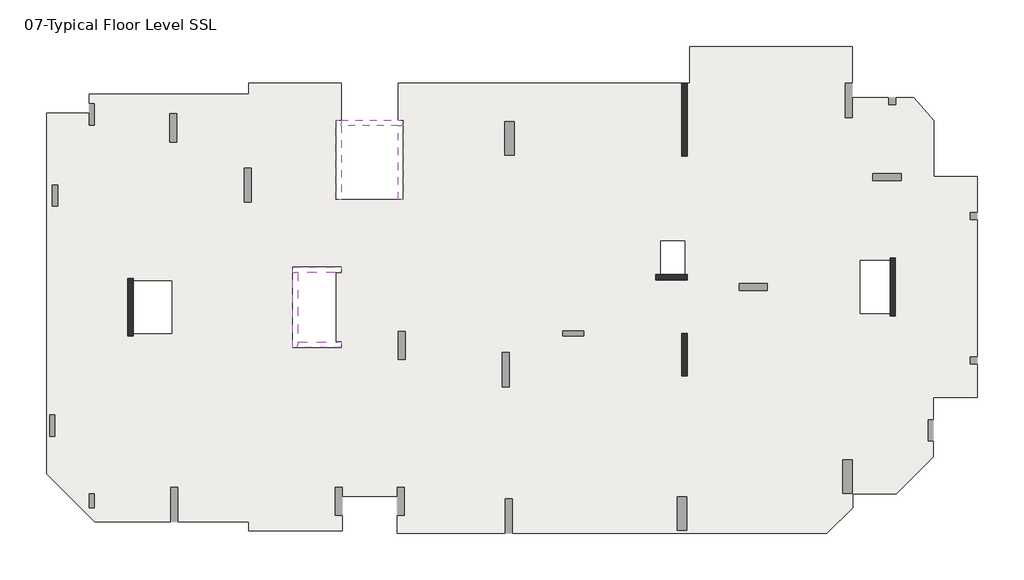
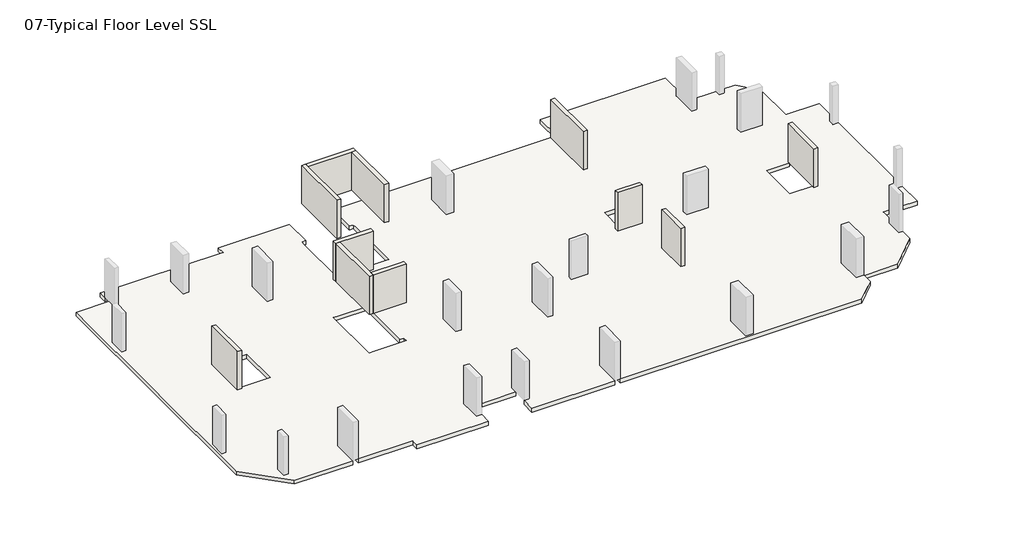
# One storey, part 1 of 2: 11 walls, 1 slab.
"""IFC4 building model written with IfcOpenShell, lengths in millimetres."""

from ifc_helpers import new_model, si_unit, origin, place, context, project, spatial, faceted_brep, element, save

model = new_model("IFC4")

# Units and contexts
model_context = context("Model", 3, world=origin())
ifc_project = project(units=[si_unit("LENGTHUNIT", "METRE", prefix="MILLI")], contexts=[model_context])

# Site, building, storey
site = spatial("IfcSite", under=ifc_project)
building = spatial("IfcBuilding", under=site)
storey = spatial("IfcBuildingStorey", under=building, Name="07-Typical Floor Level SSL", Elevation=15000.0)

# Slab
placement = place(None, origin())
element("IfcSlab", 1, ObjectType="Generic 300mm", at=placement, inside=storey, context=model_context, shape_type="Brep", body=[
    faceted_brep([(36192.0021644, 24072.000519, 14700.0), (36192.0021644, 26172.000519, 14700.0), (45446.0007483, 26172.000519, 14700.0), (45446.0007483, 24087.0, 14700.0), (45046.0007483, 24087.0, 14700.0), (45046.0007483, 22137.0, 14700.0), (45446.0007483, 22137.0, 14700.0), (45446.0007483, 23252.0000315, 14700.0), (47498.6337868, 23252.0000315, 14700.0), (47498.6337868, 22852.0, 14700.0), (47898.6337868, 22852.0, 14700.0), (47898.6337868, 23252.0000315, 14700.0), (48936.764334, 23252.0000315, 14700.0), (50076.0016214, 21956.8283806, 14700.0), (50076.0016214, 18780.0084406, 14700.0), (52549.9999998, 18780.0084406, 14700.0), (52549.9999998, 16712.0, 14700.0), (52149.9999998, 16712.0, 14700.0), (52149.9999998, 16312.0, 14700.0), (52549.9999998, 16312.0, 14700.0), (52549.9999998, 8504.0039609, 14700.0), (52149.9999998, 8504.0039609, 14700.0), (52149.9999998, 8104.0039609, 14700.0), (52549.9999998, 8104.0039609, 14700.0), (52549.9999998, 6204.0084406, 14700.0), (50046.0009271, 6204.0084406, 14700.0), (50046.0009271, 4931.9999929, 14700.0), (49746.0009271, 4931.9999929, 14700.0), (49746.0009271, 3731.9999929, 14700.0), (50046.0009271, 3731.9999929, 14700.0), (50046.0009271, 2810.5958657, 14700.0), (47943.4055804, 708.000519, 14700.0), (45456.0017287, 708.000519, 14700.0), (45456.0017287, -61.7051085, 14700.0), (43990.7023722, -1527.004465, 14700.0), (26113.9999998, -1527.004465, 14700.0), (26113.9999998, 422.995535, 14700.0), (25713.9999998, 422.995535, 14700.0), (25713.9999998, -1527.004465, 14700.0), (19569.9997488, -1527.004465, 14700.0), (19569.9997488, -512.0044652, 14700.0), (19969.9997488, -512.0044652, 14700.0), (19969.9997488, 1087.9955348, 14700.0), (19569.9997488, 1087.9955348, 14700.0), (19569.9997488, 564.000519, 14700.0), (16429.9999981, 564.000519, 14700.0), (16429.9999981, 1088.0, 14700.0), (16029.9999981, 1088.0, 14700.0), (16029.9999981, -512.0, 14700.0), (16429.9999981, -512.0, 14700.0), (16429.9999981, -1391.999481, 14700.0), (11136.0000923, -1391.999481, 14700.0), (11136.0000923, -866.9999847, 14700.0), (7082.0000416, -866.9999847, 14700.0), (7082.0000416, 1083.0000153, 14700.0), (6682.0000416, 1083.0000153, 14700.0), (6682.0000416, -866.9999847, 14700.0), (2364.4419097, -866.9999847, 14700.0), (-372.0, 1869.441925, 14700.0), (-372.0, 22380.0004589, 14700.0), (2052.0, 22380.0004589, 14700.0), (2052.0, 21708.0000656, 14700.0), (2352.0, 21708.0000656, 14700.0), (2352.0, 22908.0000656, 14700.0), (2052.0, 22908.0000656, 14700.0), (2052.0, 23472.000519, 14700.0), (11136.0000923, 23472.000519, 14700.0), (11136.0000923, 24072.000519, 14700.0), (16380.0000168, 24072.000519, 14700.0), (16380.0000168, 21972.0, 14700.0), (16079.9999997, 21972.0, 14700.0), (16079.9999997, 21672.0, 14700.0), (16079.9999997, 17468.0, 14700.0), (16379.9999997, 17468.0, 14700.0), (19619.9999997, 17468.0, 14700.0), (19919.9999997, 17468.0, 14700.0), (19919.9999997, 21672.0, 14700.0), (19919.9999997, 21972.0, 14700.0), (19619.9997365, 21972.0, 14700.0), (19619.9997365, 24072.000519, 14700.0), (35747.9999998, 24072.000519, 14700.0), (35747.9999998, 19932.0, 14700.0), (36047.9999998, 19932.0, 14700.0), (36047.9999998, 24072.000519, 14700.0), (16079.9999907, 9359.999998, 14700.0), (16079.9999907, 13320.0000002, 14700.0), (16380.0000168, 13320.0000002, 14700.0), (16380.0000168, 13620.0000002, 14700.0), (13919.9999907, 13620.0000002, 14700.0), (13619.9999907, 13620.0000002, 14700.0), (13619.9999907, 13320.0000002, 14700.0), (13619.9999907, 9359.999998, 14700.0), (13619.9999907, 9059.999998, 14700.0), (13919.9999907, 9059.999998, 14700.0), (16380.0000168, 9059.999998, 14700.0), (16380.0000168, 9359.999998, 14700.0), (4548.0000034, 9840.0000003, 14700.0), (6743.9999995, 9840.0000003, 14700.0), (6743.9999995, 12840.0000003, 14700.0), (4548.0000034, 12840.0000003, 14700.0), (4548.0000025, 12984.0000001, 14700.0), (4248.0000025, 12984.0000001, 14700.0), (4248.0000025, 9696.0, 14700.0), (4548.0000025, 9696.0, 14700.0), (47580.0014798, 13992.0079177, 14700.0), (45900.001729, 13992.0079177, 14700.0), (45900.001729, 10992.0079181, 14700.0), (47580.0014798, 10992.0079181, 14700.0), (47580.0014811, 10848.0079202, 14700.0), (47880.0014811, 10848.0079202, 14700.0), (47880.0014811, 14136.0000002, 14700.0), (47580.0014811, 14136.0000002, 14700.0), (35904.002157, 15108.0000083, 14700.0), (34548.0015145, 15108.0000083, 14700.0), (34548.0015145, 13199.9999992, 14700.0), (34248.0015201, 13199.9999992, 14700.0), (34248.0015201, 12899.9999992, 14700.0), (36048.0015201, 12899.9999992, 14700.0), (36048.0015201, 13199.9999992, 14700.0), (35904.002157, 13199.9999992, 14700.0), (257.9999999, 17088.0, 14700.0), (257.9999999, 18288.0, 14700.0), (-42.0000001, 18288.0, 14700.0), (-42.0000001, 17088.0, 14700.0), (108.001803, 4001.9999858, 14700.0), (108.001803, 5201.9999858, 14700.0), (-191.998197, 5201.9999858, 14700.0), (-191.998197, 4001.9999858, 14700.0), (30175.9999998, 9996.0000019, 14700.0), (28975.9999998, 9996.0000019, 14700.0), (28975.9999998, 9696.0000019, 14700.0), (30175.9999998, 9696.0000019, 14700.0), (7021.9999999, 20740.0000078, 14700.0), (7021.9999999, 22340.0000078, 14700.0), (6621.9999999, 22340.0000078, 14700.0), (6621.9999999, 20740.0000078, 14700.0), (48205.9993605, 18950.0, 14700.0), (46605.9993605, 18950.0, 14700.0), (46605.9993605, 18550.0, 14700.0), (48205.9993605, 18550.0, 14700.0), (20030.000009, 8355.9999979, 14700.0), (20030.000009, 9955.9999979, 14700.0), (19630.000009, 9955.9999979, 14700.0), (19630.000009, 8355.9999979, 14700.0), (11270.0000427, 17312.9999996, 14700.0), (11270.0000427, 19262.9999996, 14700.0), (10870.0000427, 19262.9999996, 14700.0), (10870.0000427, 17312.9999996, 14700.0), (40598.0014887, 12692.0079212, 14700.0), (38998.0014887, 12692.0079212, 14700.0), (38998.0014887, 12292.0079212, 14700.0), (40598.0014887, 12292.0079212, 14700.0), (2352.0, -72.0, 14700.0), (2352.0, 728.0, 14700.0), (2052.0, 728.0, 14700.0), (2052.0, -72.0, 14700.0), (25934.0000455, 6801.0001824, 14700.0), (25934.0000455, 8751.0001824, 14700.0), (25534.0000455, 8751.0001824, 14700.0), (25534.0000455, 6801.0001824, 14700.0), (36035.9999998, -1351.9992017, 14700.0), (36035.9999998, 548.0007983, 14700.0), (35485.9999998, 548.0007983, 14700.0), (35485.9999998, -1351.9992017, 14700.0), (45443.9999998, 748.0, 14700.0), (45443.9999998, 2648.0, 14700.0), (44893.9999998, 2648.0, 14700.0), (44893.9999998, 748.0, 14700.0), (26218.9999998, 20000.0, 14700.0), (26218.9999998, 21900.0, 14700.0), (25668.9999998, 21900.0, 14700.0), (25668.9999998, 20000.0, 14700.0), (35748.0054035, 9840.0000002, 14700.0), (35748.0054035, 7428.0000762, 14700.0), (36048.0054035, 7428.0000762, 14700.0), (36048.0054035, 9840.0000002, 14700.0), (36192.0021644, 26172.000519, 15000.0), (36192.0021644, 24072.000519, 15000.0), (36047.9999998, 24072.000519, 15000.0), (36047.9999998, 19932.0, 15000.0), (35747.9999998, 19932.0, 15000.0), (35747.9999998, 24072.000519, 15000.0), (19619.9997365, 24072.000519, 15000.0), (19619.9997365, 21972.0, 15000.0), (19919.9999997, 21972.0, 15000.0), (19919.9999997, 21672.0, 15000.0), (19919.9999997, 17468.0, 15000.0), (19619.9999997, 17468.0, 15000.0), (16379.9999997, 17468.0, 15000.0), (16079.9999997, 17468.0, 15000.0), (16079.9999997, 21672.0, 15000.0), (16079.9999997, 21972.0, 15000.0), (16380.0000168, 21972.0, 15000.0), (16380.0000168, 24072.000519, 15000.0), (11136.0000923, 24072.000519, 15000.0), (11136.0000923, 23472.000519, 15000.0), (2052.0, 23472.000519, 15000.0), (2052.0, 22908.0000656, 15000.0), (2352.0, 22908.0000656, 15000.0), (2352.0, 21708.0000656, 15000.0), (2052.0, 21708.0000656, 15000.0), (2052.0, 22380.0004589, 15000.0), (-372.0, 22380.0004589, 15000.0), (-372.0, 1869.441925, 15000.0), (2364.4419097, -866.9999847, 15000.0), (6682.0000416, -866.9999847, 15000.0), (6682.0000416, 1083.0000153, 15000.0), (7082.0000416, 1083.0000153, 15000.0), (7082.0000416, -866.9999847, 15000.0), (11136.0000923, -866.9999847, 15000.0), (11136.0000923, -1391.999481, 15000.0), (16429.9999981, -1391.999481, 15000.0), (16429.9999981, -512.0, 15000.0), (16029.9999981, -512.0, 15000.0), (16029.9999981, 1088.0, 15000.0), (16429.9999981, 1088.0, 15000.0), (16429.9999981, 564.000519, 15000.0), (19569.9997488, 564.000519, 15000.0), (19569.9997488, 1087.9955348, 15000.0), (19969.9997488, 1087.9955348, 15000.0), (19969.9997488, -512.0044652, 15000.0), (19569.9997488, -512.0044652, 15000.0), (19569.9997488, -1527.004465, 15000.0), (25713.9999998, -1527.004465, 15000.0), (25713.9999998, 422.995535, 15000.0), (26113.9999998, 422.995535, 15000.0), (26113.9999998, -1527.004465, 15000.0), (43990.7023722, -1527.004465, 15000.0), (45456.0017287, -61.7051085, 15000.0), (45456.0017287, 708.000519, 15000.0), (47943.4055804, 708.000519, 15000.0), (50046.0009271, 2810.5958657, 15000.0), (50046.0009271, 3731.9999929, 15000.0), (49746.0009271, 3731.9999929, 15000.0), (49746.0009271, 4931.9999929, 15000.0), (50046.0009271, 4931.9999929, 15000.0), (50046.0009271, 6204.0084406, 15000.0), (52549.9999998, 6204.0084406, 15000.0), (52549.9999998, 8104.0039609, 15000.0), (52149.9999998, 8104.0039609, 15000.0), (52149.9999998, 8504.0039609, 15000.0), (52549.9999998, 8504.0039609, 15000.0), (52549.9999998, 16312.0, 15000.0), (52149.9999998, 16312.0, 15000.0), (52149.9999998, 16712.0, 15000.0), (52549.9999998, 16712.0, 15000.0), (52549.9999998, 18780.0084406, 15000.0), (50076.0016214, 18780.0084406, 15000.0), (50076.0016214, 21956.8283806, 15000.0), (48936.764334, 23252.0000315, 15000.0), (47898.6337868, 23252.0000315, 15000.0), (47898.6337868, 22852.0, 15000.0), (47498.6337868, 22852.0, 15000.0), (47498.6337868, 23252.0000315, 15000.0), (45446.0006898, 23252.0000315, 15000.0), (45446.0007483, 22137.0, 15000.0), (45046.0007483, 22137.0, 15000.0), (45046.0007483, 24087.0, 15000.0), (45446.0007483, 24087.0, 15000.0), (45446.0007483, 26172.000519, 15000.0), (16079.9999907, 13320.0000002, 15000.0), (16079.9999907, 9359.999998, 15000.0), (16380.0000168, 9359.999998, 15000.0), (16380.0000168, 9059.999998, 15000.0), (13919.9999907, 9059.999998, 15000.0), (13619.9999907, 9059.999998, 15000.0), (13619.9999907, 9359.999998, 15000.0), (13619.9999907, 13320.0000002, 15000.0), (13619.9999907, 13620.0000002, 15000.0), (13919.9999907, 13620.0000002, 15000.0), (16380.0000168, 13620.0000002, 15000.0), (16380.0000168, 13320.0000002, 15000.0), (6743.9999995, 9840.0000003, 15000.0), (4548.0000034, 9840.0000003, 15000.0), (4548.0000025, 9696.0, 15000.0), (4248.0000025, 9696.0, 15000.0), (4248.0000025, 12984.0000001, 15000.0), (4548.0000025, 12984.0000001, 15000.0), (4548.0000025, 12840.0000003, 15000.0), (6743.9999995, 12840.0000003, 15000.0), (45900.001729, 13992.0079177, 15000.0), (47580.0014798, 13992.0079177, 15000.0), (47580.0014811, 14136.0000002, 15000.0), (47880.0014811, 14136.0000002, 15000.0), (47880.0014811, 10848.0079202, 15000.0), (47580.0014811, 10848.0079202, 15000.0), (47580.0014811, 10992.0079181, 15000.0), (45900.001729, 10992.0079181, 15000.0), (34548.0015145, 15108.0000083, 15000.0), (35904.002157, 15108.0000083, 15000.0), (35904.002157, 13199.9999992, 15000.0), (36048.0015201, 13199.9999992, 15000.0), (36048.0015201, 12899.9999992, 15000.0), (34248.0015201, 12899.9999992, 15000.0), (34248.0015201, 13199.9999992, 15000.0), (34548.0015145, 13199.9999992, 15000.0), (257.9999999, 18288.0, 15000.0), (257.9999999, 17088.0, 15000.0), (-42.0000001, 17088.0, 15000.0), (-42.0000001, 18288.0, 15000.0), (108.001803, 5201.9999858, 15000.0), (108.001803, 4001.9999858, 15000.0), (-191.998197, 4001.9999858, 15000.0), (-191.998197, 5201.9999858, 15000.0), (28975.9999998, 9996.0000019, 15000.0), (30175.9999998, 9996.0000019, 15000.0), (30175.9999998, 9696.0000019, 15000.0), (28975.9999998, 9696.0000019, 15000.0), (7021.9999999, 22340.0000078, 15000.0), (7021.9999999, 20740.0000078, 15000.0), (6621.9999999, 20740.0000078, 15000.0), (6621.9999999, 22340.0000078, 15000.0), (46605.9993605, 18950.0, 15000.0), (48205.9993605, 18950.0, 15000.0), (48205.9993605, 18550.0, 15000.0), (46605.9993605, 18550.0, 15000.0), (20030.000009, 9955.9999979, 15000.0), (20030.000009, 8355.9999979, 15000.0), (19630.000009, 8355.9999979, 15000.0), (19630.000009, 9955.9999979, 15000.0), (11270.0000427, 19262.9999996, 15000.0), (11270.0000427, 17312.9999996, 15000.0), (10870.0000427, 17312.9999996, 15000.0), (10870.0000427, 19262.9999996, 15000.0), (38998.0014887, 12692.0079212, 15000.0), (40598.0014887, 12692.0079212, 15000.0), (40598.0014887, 12292.0079212, 15000.0), (38998.0014887, 12292.0079212, 15000.0), (2352.0, 728.0, 15000.0), (2352.0, -72.0, 15000.0), (2052.0, -72.0, 15000.0), (2052.0, 728.0, 15000.0), (25934.0000455, 8751.0001824, 15000.0), (25934.0000455, 6801.0001824, 15000.0), (25534.0000455, 6801.0001824, 15000.0), (25534.0000455, 8751.0001824, 15000.0), (36035.9999998, 548.0007983, 15000.0), (36035.9999998, -1351.9992017, 15000.0), (35485.9999998, -1351.9992017, 15000.0), (35485.9999998, 548.0007983, 15000.0), (45443.9999998, 2648.0, 15000.0), (45443.9999998, 748.0, 15000.0), (44893.9999998, 748.0, 15000.0), (44893.9999998, 2648.0, 15000.0), (26218.9999998, 21900.0, 15000.0), (26218.9999998, 20000.0, 15000.0), (25668.9999998, 20000.0, 15000.0), (25668.9999998, 21900.0, 15000.0), (35748.0054035, 7428.0000762, 15000.0), (35748.0054035, 9840.0000002, 15000.0), (36048.0054035, 9840.0000002, 15000.0), (36048.0054035, 7428.0000762, 15000.0)], [[[0, 1, 2, 3, 4, 5, 6, 7, 8, 9, 10, 11, 12, 13, 14, 15, 16, 17, 18, 19, 20, 21, 22, 23, 24, 25, 26, 27, 28, 29, 30, 31, 32, 33, 34, 35, 36, 37, 38, 39, 40, 41, 42, 43, 44, 45, 46, 47, 48, 49, 50, 51, 52, 53, 54, 55, 56, 57, 58, 59, 60, 61, 62, 63, 64, 65, 66, 67, 68, 69, 70, 71, 72, 73, 74, 75, 76, 77, 78, 79, 80, 81, 82, 83], [84, 85, 86, 87, 88, 89, 90, 91, 92, 93, 94, 95], [96, 97, 98, 99, 100, 101, 102, 103], [104, 105, 106, 107, 108, 109, 110, 111], [112, 113, 114, 115, 116, 117, 118, 119], [120, 121, 122, 123], [124, 125, 126, 127], [128, 129, 130, 131], [132, 133, 134, 135], [136, 137, 138, 139], [140, 141, 142, 143], [144, 145, 146, 147], [148, 149, 150, 151], [152, 153, 154, 155], [156, 157, 158, 159], [160, 161, 162, 163], [164, 165, 166, 167], [168, 169, 170, 171], [172, 173, 174, 175]], [[176, 177, 178, 179, 180, 181, 182, 183, 184, 185, 186, 187, 188, 189, 190, 191, 192, 193, 194, 195, 196, 197, 198, 199, 200, 201, 202, 203, 204, 205, 206, 207, 208, 209, 210, 211, 212, 213, 214, 215, 216, 217, 218, 219, 220, 221, 222, 223, 224, 225, 226, 227, 228, 229, 230, 231, 232, 233, 234, 235, 236, 237, 238, 239, 240, 241, 242, 243, 244, 245, 246, 247, 248, 249, 250, 251, 252, 253, 254, 255, 256, 257, 258, 259], [260, 261, 262, 263, 264, 265, 266, 267, 268, 269, 270, 271], [272, 273, 274, 275, 276, 277, 278, 279], [280, 281, 282, 283, 284, 285, 286, 287], [288, 289, 290, 291, 292, 293, 294, 295], [296, 297, 298, 299], [300, 301, 302, 303], [304, 305, 306, 307], [308, 309, 310, 311], [312, 313, 314, 315], [316, 317, 318, 319], [320, 321, 322, 323], [324, 325, 326, 327], [328, 329, 330, 331], [332, 333, 334, 335], [336, 337, 338, 339], [340, 341, 342, 343], [344, 345, 346, 347], [348, 349, 350, 351]], [[68, 193, 192, 69]], [[182, 79, 78, 183]], [[79, 182, 181, 80]], [[177, 0, 83, 178]], [[1, 0, 177, 176]], [[2, 1, 176, 259]], [[3, 2, 259, 258]], [[249, 12, 11, 250]], [[7, 254, 253, 8]], [[13, 12, 249, 248]], [[14, 13, 248, 247]], [[15, 14, 247, 246]], [[15, 246, 245, 16]], [[237, 24, 23, 238]], [[19, 242, 241, 20]], [[25, 24, 237, 236]], [[25, 236, 235, 26]], [[231, 30, 29, 232]], [[32, 31, 230, 229]], [[33, 32, 229, 228]], [[34, 33, 228, 227]], [[34, 227, 226, 35]], [[222, 39, 38, 223]], [[39, 222, 221, 40]], [[45, 44, 217, 216]], [[211, 50, 49, 212]], [[51, 50, 211, 210]], [[52, 51, 210, 209]], [[52, 209, 208, 53]], [[204, 57, 56, 205]], [[58, 57, 204, 203]], [[59, 58, 203, 202]], [[60, 59, 202, 201]], [[196, 65, 64, 197]], [[66, 65, 196, 195]], [[67, 66, 195, 194]], [[68, 67, 194, 193]], [[31, 30, 231, 230]], [[85, 84, 261, 260]], [[72, 189, 188, 187, 186, 75, 74, 73]], [[272, 97, 96, 273]], [[97, 272, 279, 98]], [[98, 279, 278, 99]], [[280, 105, 104, 281]], [[105, 280, 287, 106]], [[106, 287, 286, 107]], [[112, 289, 288, 113]], [[113, 288, 295, 114]], [[289, 112, 119, 290]], [[62, 199, 198, 63]], [[199, 62, 61, 200]], [[200, 61, 60, 201]], [[63, 198, 197, 64]], [[120, 297, 296, 121]], [[297, 120, 123, 298]], [[298, 123, 122, 299]], [[299, 122, 121, 296]], [[124, 301, 300, 125]], [[301, 124, 127, 302]], [[302, 127, 126, 303]], [[303, 126, 125, 300]], [[28, 233, 232, 29]], [[233, 28, 27, 234]], [[234, 27, 26, 235]], [[128, 305, 304, 129]], [[305, 128, 131, 306]], [[306, 131, 130, 307]], [[307, 130, 129, 304]], [[132, 309, 308, 133]], [[309, 132, 135, 310]], [[310, 135, 134, 311]], [[311, 134, 133, 308]], [[41, 220, 219, 42]], [[220, 41, 40, 221]], [[43, 218, 217, 44]], [[218, 43, 42, 219]], [[136, 313, 312, 137]], [[313, 136, 139, 314]], [[314, 139, 138, 315]], [[315, 138, 137, 312]], [[140, 317, 316, 141]], [[317, 140, 143, 318]], [[318, 143, 142, 319]], [[319, 142, 141, 316]], [[215, 46, 45, 216]], [[48, 213, 212, 49]], [[213, 48, 47, 214]], [[214, 47, 46, 215]], [[144, 321, 320, 145]], [[321, 144, 147, 322]], [[322, 147, 146, 323]], [[323, 146, 145, 320]], [[207, 54, 53, 208]], [[55, 206, 205, 56]], [[206, 55, 54, 207]], [[225, 36, 35, 226]], [[37, 224, 223, 38]], [[224, 37, 36, 225]], [[6, 255, 254, 7]], [[255, 6, 5, 256]], [[256, 5, 4, 257]], [[257, 4, 3, 258]], [[148, 325, 324, 149]], [[325, 148, 151, 326]], [[326, 151, 150, 327]], [[327, 150, 149, 324]], [[152, 329, 328, 153]], [[329, 152, 155, 330]], [[330, 155, 154, 331]], [[331, 154, 153, 328]], [[156, 333, 332, 157]], [[333, 156, 159, 334]], [[334, 159, 158, 335]], [[335, 158, 157, 332]], [[160, 337, 336, 161]], [[337, 160, 163, 338]], [[338, 163, 162, 339]], [[339, 162, 161, 336]], [[164, 341, 340, 165]], [[341, 164, 167, 342]], [[342, 167, 166, 343]], [[343, 166, 165, 340]], [[168, 345, 344, 169]], [[345, 168, 171, 346]], [[346, 171, 170, 347]], [[347, 170, 169, 344]], [[70, 191, 190, 189, 72, 71]], [[191, 70, 69, 192]], [[77, 184, 183, 78]], [[184, 77, 76, 75, 186, 185]], [[271, 86, 85, 260]], [[87, 270, 269, 268, 89, 88]], [[86, 271, 270, 87]], [[89, 268, 267, 266, 265, 92, 91, 90]], [[92, 265, 264, 263, 94, 93]], [[95, 262, 261, 84]], [[262, 95, 94, 263]], [[277, 100, 99, 278]], [[103, 274, 273, 96]], [[101, 276, 275, 102]], [[100, 277, 276, 101]], [[274, 103, 102, 275]], [[116, 293, 292, 117]], [[118, 291, 290, 119]], [[294, 115, 114, 295]], [[117, 292, 291, 118]], [[293, 116, 115, 294]], [[172, 349, 348, 173]], [[174, 351, 350, 175]], [[173, 348, 351, 174]], [[349, 172, 175, 350]], [[285, 108, 107, 286]], [[111, 282, 281, 104]], [[109, 284, 283, 110]], [[108, 285, 284, 109]], [[282, 111, 110, 283]], [[82, 179, 178, 83]], [[180, 81, 80, 181]], [[179, 82, 81, 180]], [[18, 243, 242, 19]], [[243, 18, 17, 244]], [[244, 17, 16, 245]], [[10, 251, 250, 11]], [[251, 10, 9, 252]], [[252, 9, 8, 253]], [[22, 239, 238, 23]], [[239, 22, 21, 240]], [[240, 21, 20, 241]]]),
])

# Walls
element("IfcWall", 2, ObjectType="Shear Walls 300mm", at=placement, inside=storey, context=model_context, shape_type="Brep", body=[
    faceted_brep([(4548.0000025, 9696.0, 15000.0), (4548.0000025, 12984.0000001, 15000.0), (4548.0000025, 12984.0000001, 17700.0), (4548.0000025, 12984.0000001, 18000.0), (4548.0000025, 12840.0000003, 18000.0), (4548.0000025, 9840.0000003, 18000.0), (4548.0000025, 9696.0, 18000.0), (4548.0000025, 9696.0, 17700.0), (4248.0000025, 9696.0, 15000.0), (4248.0000025, 9696.0, 17700.0), (4248.0000025, 9696.0, 18000.0), (4248.0000025, 12984.0000001, 18000.0), (4248.0000025, 12984.0000001, 17700.0), (4248.0000025, 12984.0000001, 15000.0)], [[[0, 1, 2, 3, 4, 5, 6, 7]], [[8, 9, 10, 11, 12, 13]], [[1, 0, 8, 13]], [[3, 2, 1, 13, 12, 11]], [[6, 5, 4, 3, 11, 10]], [[0, 7, 6, 10, 9, 8]]]),
])
element("IfcWall", 3, ObjectType="Shear Walls 300mm", at=placement, inside=storey, context=model_context, shape_type="Brep", body=[
    faceted_brep([(34248.0015201, 12899.9999992, 15000.0), (36048.0015201, 12899.9999992, 15000.0), (36048.0015201, 12899.9999992, 17700.0), (36048.0015201, 12899.9999992, 18000.0), (34248.0015201, 12899.9999992, 18000.0), (34248.0015201, 12899.9999992, 17700.0), (34248.0015201, 13199.9999992, 15000.0), (34248.0015201, 13199.9999992, 17700.0), (34248.0015201, 13199.9999992, 18000.0), (34548.0015145, 13199.9999992, 18000.0), (35904.002157, 13199.9999992, 18000.0), (36048.0015201, 13199.9999992, 18000.0), (36048.0015201, 13199.9999992, 17700.0), (36048.0015201, 13199.9999992, 15000.0)], [[[0, 1, 2, 3, 4, 5]], [[6, 7, 8, 9, 10, 11, 12, 13]], [[1, 0, 6, 13]], [[3, 2, 1, 13, 12, 11]], [[4, 3, 11, 10, 9, 8]], [[0, 5, 4, 8, 7, 6]]]),
])
element("IfcWall", 4, ObjectType="Shear Walls 300mm", at=placement, inside=storey, context=model_context, shape_type="Brep", body=[
    faceted_brep([(35748.0054035, 9840.0000002, 15000.0), (35748.0054035, 7428.0000762, 15000.0), (35748.0054035, 7428.0000762, 17700.0), (35748.0054035, 7428.0000762, 18000.0), (35748.0054035, 9840.0000002, 18000.0), (35748.0054035, 9840.0000002, 17700.0), (36048.0054035, 9840.0000002, 15000.0), (36048.0054035, 9840.0000002, 17700.0), (36048.0054035, 9840.0000002, 18000.0), (36048.0054035, 7428.0000762, 18000.0), (36048.0054035, 7428.0000762, 17700.0), (36048.0054035, 7428.0000762, 15000.0)], [[[0, 1, 2, 3, 4, 5]], [[6, 7, 8, 9, 10, 11]], [[1, 0, 6, 11]], [[3, 2, 1, 11, 10, 9]], [[4, 3, 9, 8]], [[0, 5, 4, 8, 7, 6]]]),
])
element("IfcWall", 5, ObjectType="Shear Walls 300mm", at=placement, inside=storey, context=model_context, shape_type="Brep", body=[
    faceted_brep([(47580.0014811, 14136.0000002, 15000.0), (47580.0014811, 10848.0079202, 15000.0), (47580.0014811, 10848.0079202, 17700.0), (47580.0014811, 10848.0079202, 18000.0), (47580.0014811, 10992.0079181, 18000.0), (47580.0014811, 13992.0079177, 18000.0), (47580.0014811, 14136.0000002, 18000.0), (47580.0014811, 14136.0000002, 17700.0), (47880.0014811, 14136.0000002, 15000.0), (47880.0014811, 14136.0000002, 17700.0), (47880.0014811, 14136.0000002, 18000.0), (47880.0014811, 10848.0079202, 18000.0), (47880.0014811, 10848.0079202, 17700.0), (47880.0014811, 10848.0079202, 15000.0)], [[[0, 1, 2, 3, 4, 5, 6, 7]], [[8, 9, 10, 11, 12, 13]], [[1, 0, 8, 13]], [[3, 2, 1, 13, 12, 11]], [[6, 5, 4, 3, 11, 10]], [[0, 7, 6, 10, 9, 8]]]),
])
element("IfcWall", 6, ObjectType="Shear Walls 300mm", at=placement, inside=storey, context=model_context, shape_type="Brep", body=[
    faceted_brep([(36047.9999998, 19932.0, 15000.0), (36047.9999998, 24072.0078999, 15000.0), (36047.9999998, 24072.0078999, 18000.0), (36047.9999998, 19932.0, 18000.0), (36047.9999998, 19932.0, 17700.0), (35747.9999998, 19932.0, 15000.0), (35747.9999998, 19932.0, 17700.0), (35747.9999998, 19932.0, 18000.0), (35747.9999998, 24072.0078999, 18000.0), (35747.9999998, 24072.0078999, 15000.0)], [[[0, 1, 2, 3, 4]], [[5, 6, 7, 8, 9]], [[1, 0, 5, 9]], [[2, 1, 9, 8]], [[3, 2, 8, 7]], [[0, 4, 3, 7, 6, 5]]]),
])
element("IfcWall", 7, ObjectType="Shear Walls 300mm", at=placement, inside=storey, context=model_context, shape_type="Brep", body=[
    faceted_brep([(16379.9999997, 21972.0, 21000.0), (16379.9999997, 21672.0, 21000.0), (16379.9999997, 17468.0, 21000.0), (16379.9999997, 17468.0, 18000.0), (16379.9999997, 21672.0, 18000.0), (16379.9999997, 21972.0, 18000.0), (16079.9999997, 17468.0, 21000.0), (16079.9999997, 21972.0, 21000.0), (16079.9999997, 21972.0, 20700.0), (16079.9999997, 21972.0, 18000.0), (16079.9999997, 17468.0, 18000.0), (16079.9999997, 17468.0, 20700.0)], [[[0, 1, 2, 3, 4, 5]], [[6, 7, 8, 9, 10, 11]], [[2, 1, 0, 7, 6]], [[2, 6, 11, 10, 3]], [[3, 10, 9, 5, 4]], [[0, 5, 9, 8, 7]]]),
])
element("IfcWall", 8, ObjectType="Shear Walls 300mm", at=placement, inside=storey, context=model_context, shape_type="Brep", body=[
    faceted_brep([(16379.9999997, 21972.0, 21000.0), (19619.9997365, 21972.0, 21000.0), (19919.9999997, 21972.0, 21000.0), (19919.9999997, 21972.0, 20700.0), (19919.9999997, 21972.0, 18000.0), (16379.9999997, 21972.0, 18000.0), (19919.9999997, 21672.0, 21000.0), (19619.9999997, 21672.0, 21000.0), (16379.9999997, 21672.0, 21000.0), (16379.9999997, 21672.0, 18000.0), (19619.9999997, 21672.0, 18000.0), (19919.9999997, 21672.0, 18000.0)], [[[0, 1, 2, 3, 4, 5]], [[6, 7, 8, 9, 10, 11]], [[2, 1, 0, 8, 7, 6]], [[8, 0, 5, 9]], [[9, 5, 4, 11, 10]], [[4, 3, 2, 6, 11]]]),
])
element("IfcWall", 9, ObjectType="Shear Walls 300mm", at=placement, inside=storey, context=model_context, shape_type="Brep", body=[
    faceted_brep([(19919.9999997, 21672.0, 21000.0), (19919.9999997, 17468.0, 21000.0), (19919.9999997, 17468.0, 20700.0), (19919.9999997, 17468.0, 18000.0), (19919.9999997, 21672.0, 18000.0), (19619.9999997, 17468.0, 21000.0), (19619.9999997, 21672.0, 21000.0), (19619.9999997, 21672.0, 18000.0), (19619.9999997, 17468.0, 18000.0)], [[[0, 1, 2, 3, 4]], [[5, 6, 7, 8]], [[1, 0, 6, 5]], [[1, 5, 8, 3, 2]], [[6, 0, 4, 7]], [[4, 3, 8, 7]]]),
])
element("IfcWall", 10, ObjectType="Shear Walls 300mm", at=placement, inside=storey, context=model_context, shape_type="Brep", body=[
    faceted_brep([(16380.0000168, 13320.0000002, 21000.0), (16079.9999907, 13320.0000002, 21000.0), (13919.9999907, 13320.0000002, 21000.0), (13619.9999907, 13320.0000002, 21000.0), (13619.9999907, 13320.0000002, 18000.0), (13919.9999907, 13320.0000002, 18000.0), (16380.0000168, 13320.0000002, 18000.0), (16380.0000168, 13320.0000002, 20700.0), (13619.9999907, 13620.0000002, 21000.0), (16380.0000168, 13620.0000002, 21000.0), (16380.0000168, 13620.0000002, 20700.0), (16380.0000168, 13620.0000002, 18000.0), (13619.9999907, 13620.0000002, 18000.0), (13619.9999907, 13620.0000002, 20700.0)], [[[0, 1, 2, 3, 4, 5, 6, 7]], [[8, 9, 10, 11, 12, 13]], [[9, 0, 7, 6, 11, 10]], [[3, 2, 1, 0, 9, 8]], [[11, 6, 5, 4, 12]], [[4, 3, 8, 13, 12]]]),
])
element("IfcWall", 11, ObjectType="Shear Walls 300mm", at=placement, inside=storey, context=model_context, shape_type="Brep", body=[
    faceted_brep([(13919.9999907, 13320.0000002, 21000.0), (13919.9999907, 9359.999998, 21000.0), (13919.9999907, 9059.999998, 21000.0), (13919.9999907, 9059.999998, 18000.0), (13919.9999907, 9359.999998, 18000.0), (13919.9999907, 13320.0000002, 18000.0), (13619.9999907, 9059.999998, 21000.0), (13619.9999907, 13320.0000002, 21000.0), (13619.9999907, 13320.0000002, 18000.0), (13619.9999907, 9059.999998, 18000.0), (13619.9999907, 9059.999998, 20700.0)], [[[0, 1, 2, 3, 4, 5]], [[6, 7, 8, 9, 10]], [[2, 1, 0, 7, 6]], [[7, 0, 5, 8]], [[8, 5, 4, 3, 9]], [[3, 2, 6, 10, 9]]]),
])
element("IfcWall", 12, ObjectType="Shear Walls 300mm", at=placement, inside=storey, context=model_context, shape_type="Brep", body=[
    faceted_brep([(13919.9999907, 9359.999998, 21000.0), (16079.9999907, 9359.999998, 21000.0), (16380.0000168, 9359.999998, 21000.0), (16380.0000168, 9359.999998, 20700.0), (16380.0000168, 9359.999998, 18000.0), (13919.9999907, 9359.999998, 18000.0), (16380.0000168, 9059.999998, 21000.0), (13919.9999907, 9059.999998, 21000.0), (13919.9999907, 9059.999998, 18000.0), (16380.0000168, 9059.999998, 18000.0), (16380.0000168, 9059.999998, 20700.0)], [[[0, 1, 2, 3, 4, 5]], [[6, 7, 8, 9, 10]], [[2, 1, 0, 7, 6]], [[2, 6, 10, 9, 4, 3]], [[7, 0, 5, 8]], [[5, 4, 9, 8]]]),
])

save(model, "model.ifc")

# Revit data of these elements
# Type "Generic 300mm"
#   Function = 0
#   Layers, outside or top first: 300 mm "Concrete-RC" (function 1)
# Type "Shear Walls 300mm"
#   Layers, outside or top first: 300 mm "Concrete-RC" (function 1)
# Element 1 (IfcSlab, "Generic 300mm")
#   Height Offset From Level = 0 mm
#   built-in parameter 1001954 = 1
#   Phase Created = New Construction
#   Materials on its faces: "Concrete-RC"
# Elements 2, 3, 4, 5, 6 (IfcWall, "Shear Walls 300mm")
#   Top Offset = 0 mm
#   Base Offset = 0 mm
#   wall height = 3000 mm
#   Phase Created = New Construction
#   Base Constraint = 07-Typical Floor Level SSL
#   Top Constraint = 08-Typical Floor Level SSL
#   Materials on its faces: "Concrete-RC"
# Elements 7, 8, 9, 10, 11, 12 (IfcWall, "Shear Walls 300mm")
#   Top Offset = 0 mm
#   Base Offset = 0 mm
#   wall height = 6000 mm
#   Phase Created = New Construction
#   Base Constraint = 07-Typical Floor Level SSL
#   Top Constraint = 09-Typical Floor Level SSL
#   Materials on its faces: "Concrete-RC"
# Materials
#   "Concrete-RC": class "Concrete", colour RGB 128 128 128, transparency 0, Description = "High strength concrete", Cost = 0
